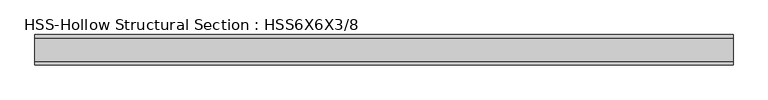
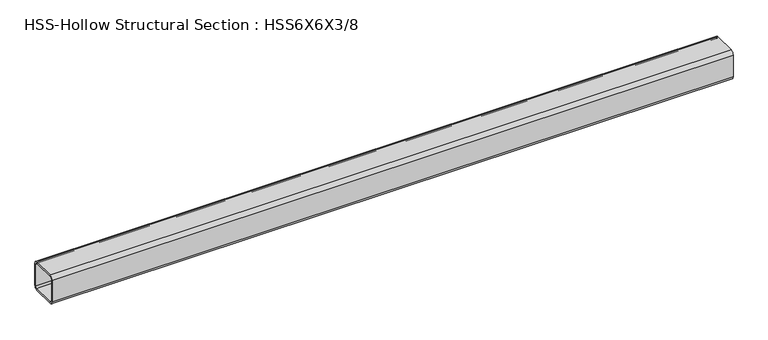
"""IFC4 building model written with IfcOpenShell, lengths in millimetres: beam geometry, HSS-Hollow Structural Section : HSS6X6X3/8."""

from ifc_helpers import new_model, si_unit, point, frame, frame_2d, origin, place, context, project, spatial, polyline, circle_curve, trimmed, segment, composite_curve, outline, extrude, source, transform, mapped, element, save


def hss_hollow_structural_section_hss6x6x3_8_2d7e4dc7(model_context):
    return source(origin(), model_context, "Body", "SweptSolid", [
        extrude(outline(composite_curve([segment(polyline([(76.2, 58.4708), (76.2, -58.4708)]), True, "CONTINUOUS"), segment(trimmed(circle_curve(frame_2d((58.4708, -58.4708)), 17.7292), [point((76.2, -58.4708))], [point((58.4708, -76.2))], False, "CARTESIAN"), True, "CONTINUOUS"), segment(polyline([(58.4708, -76.2), (-58.4708, -76.2)]), True, "CONTINUOUS"), segment(trimmed(circle_curve(frame_2d((-58.4708, -58.4708)), 17.7292), [point((-58.4708, -76.2))], [point((-76.2, -58.4708))], False, "CARTESIAN"), True, "CONTINUOUS"), segment(polyline([(-76.2, -58.4708), (-76.2, 58.4708)]), True, "CONTINUOUS"), segment(trimmed(circle_curve(frame_2d((-58.4708, 58.4708)), 17.7292), [point((-76.2, 58.4708))], [point((-58.4708, 76.2))], False, "CARTESIAN"), True, "CONTINUOUS"), segment(polyline([(-58.4708, 76.2), (58.4708, 76.2)]), True, "CONTINUOUS"), segment(trimmed(circle_curve(frame_2d((58.4708, 58.4708)), 17.7292), [point((58.4708, 76.2))], [point((76.2, 58.4708))], False, "CARTESIAN"), True, "CONTINUOUS")], self_intersect=False), holes=[composite_curve([segment(trimmed(circle_curve(frame_2d((-58.4708, 58.4708)), 8.8646), [point((-58.4708, 67.3354))], [point((-67.3354, 58.4708))], True, "CARTESIAN"), True, "CONTINUOUS"), segment(polyline([(-67.3354, 58.4708), (-67.3354, -58.4708)]), True, "CONTINUOUS"), segment(trimmed(circle_curve(frame_2d((-58.4708, -58.4708)), 8.8646), [point((-67.3354, -58.4708))], [point((-58.4708, -67.3354))], True, "CARTESIAN"), True, "CONTINUOUS"), segment(polyline([(-58.4708, -67.3354), (58.4708, -67.3354)]), True, "CONTINUOUS"), segment(trimmed(circle_curve(frame_2d((58.4708, -58.4708)), 8.8646), [point((58.4708, -67.3354))], [point((67.3354, -58.4708))], True, "CARTESIAN"), True, "CONTINUOUS"), segment(polyline([(67.3354, -58.4708), (67.3354, 58.4708)]), True, "CONTINUOUS"), segment(trimmed(circle_curve(frame_2d((58.4708, 58.4708)), 8.8646), [point((67.3354, 58.4708))], [point((58.4708, 67.3354))], True, "CARTESIAN"), True, "CONTINUOUS"), segment(polyline([(58.4708, 67.3354), (-58.4708, 67.3354)]), True, "CONTINUOUS")], self_intersect=False)]), frame((-1739.8999994, 0.0, 0.0), z_axis=(1.0, 0.0, 0.0), x_axis=(0.0, 1.0, 0.0)), (0.0, 0.0, 1.0), 3492.4999994),
    ])


if __name__ == "__main__":
    model = new_model("IFC4")
    model_context = context("Model", 3, world=origin())
    ifc_project = project(units=[si_unit("LENGTHUNIT", "METRE", prefix="MILLI")], contexts=[model_context])
    site = spatial("IfcSite", under=ifc_project)
    building = spatial("IfcBuilding", under=site)
    placement = place(None, origin())
    hss_hollow_structural_section_hss6x6x3_8_shape = hss_hollow_structural_section_hss6x6x3_8_2d7e4dc7(model_context)
    element("IfcBeam", 1, ObjectType="HSS-Hollow Structural Section : HSS6X6X3/8", at=placement, inside=building, context=model_context, shape_type="MappedRepresentation", body=[
        mapped(hss_hollow_structural_section_hss6x6x3_8_shape, transform((0.0, 0.0, 0.0), x_axis=(1.0, 0.0, 0.0), y_axis=(0.0, 1.0, 0.0), z_axis=(0.0, 0.0, 1.0))),
    ])
    save(model, "model.ifc")

# Revit data of these elements
# Type "HSS-Hollow Structural Section : HSS6X6X3/8"
#   Assembly Code = "B10"
#   Shape = "Square"
#   W = 27.4
#   Ht = 0' - 6"
#   Length [instance default] = 5' - 0"
#   b = 0' - 6"
#   kr = 0' - 0.698"
#   t = 0' - 0.349"
#   A = 0.0526389 SF
#   Structural Material [instance default] = Steel ASTM A500, Grade B, Rectangular and Square
# Element 1 (IfcBeam, "HSS-Hollow Structural Section : HSS6X6X3/8")
#   Materials on its faces: "Steel ASTM A500, Grade B, Rectangular and Square"
# Materials
#   "Steel ASTM A500, Grade B, Rectangular and Square": class "Metal", colour RGB 199 199 199, transparency 0, Description = "Carbon steel", Cost = 0
